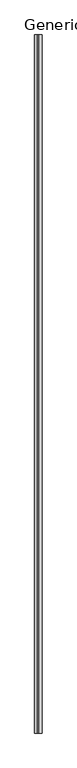
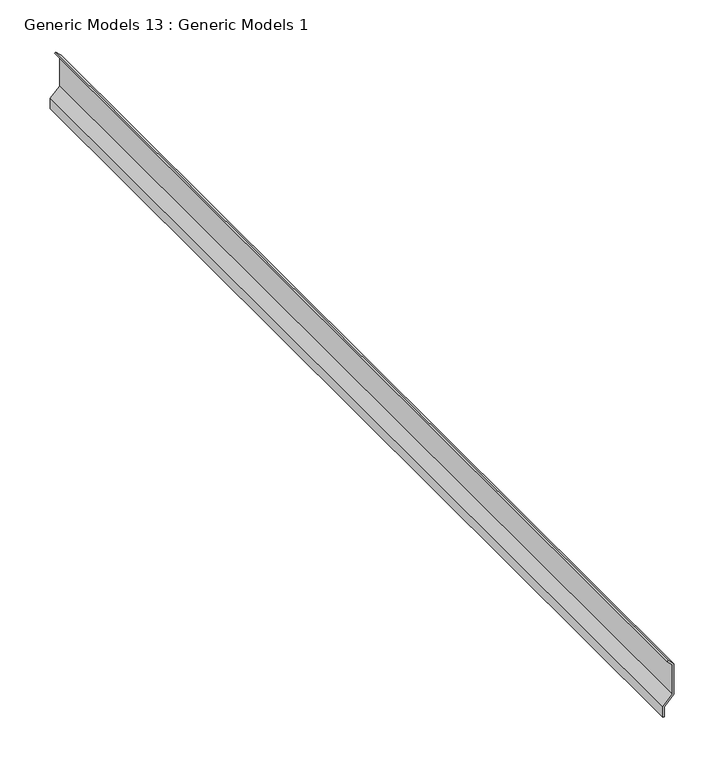
"""IFC4 building model written with IfcOpenShell, lengths in millimetres: proxy geometry, Generic Models 13 : Generic Models 1."""

from ifc_helpers import new_model, si_unit, frame, origin, place, context, project, spatial, polyline, outline, extrude, source, transform, mapped, element, save


def generic_models_13_generic_models_1_1f047596(model_context):
    return source(origin(), model_context, "Body", "SweptSolid", [
        extrude(outline(polyline([(39.3342783, 51003.2), (26.6342783, 51003.2), (26.6342783, 51004.7875), (38.6767142, 51004.7875), (49.7892142, 51015.9), (86.9592783, 51015.9), (93.3092783, 51009.55), (92.1867462, 51008.427468), (86.3017142, 51014.3125), (50.4467783, 51014.3125), (39.3342783, 51003.2)])), frame((0.0, 0.0, 0.0), z_axis=(0.0, 1.0, 0.0), x_axis=(0.0, 0.0, 1.0)), (0.0, 0.0, 1.0), 1219.2),
    ])


if __name__ == "__main__":
    model = new_model("IFC4")
    model_context = context("Model", 3, world=origin())
    ifc_project = project(units=[si_unit("LENGTHUNIT", "METRE", prefix="MILLI")], contexts=[model_context])
    site = spatial("IfcSite", under=ifc_project)
    building = spatial("IfcBuilding", under=site)
    placement = place(None, origin())
    generic_models_13_generic_models_1_shape = generic_models_13_generic_models_1_1f047596(model_context)
    element("IfcBuildingElementProxy", 1, Name="Generic Models 13 : Generic Models 1", ObjectType="Generic Models 13 : Generic Models 1", at=placement, inside=building, context=model_context, shape_type="MappedRepresentation", body=[
        mapped(generic_models_13_generic_models_1_shape, transform((0.0, 0.0, 0.0), x_axis=(1.0, 0.0, 0.0), y_axis=(0.0, 1.0, 0.0), z_axis=(0.0, 0.0, 1.0))),
    ])
    save(model, "model.ifc")

# Revit data of these elements
# Element 1 (IfcBuildingElementProxy, "Generic Models 13 : Generic Models 1")
#   Materials on its faces: "RESILIENT CHANNELS @ 2'-0\""
# Materials
#   "RESILIENT CHANNELS @ 2'-0\"": class "Metal", colour RGB 189 187 185, transparency 0, Description = "Structural steel 50ksi", Cost = 0
